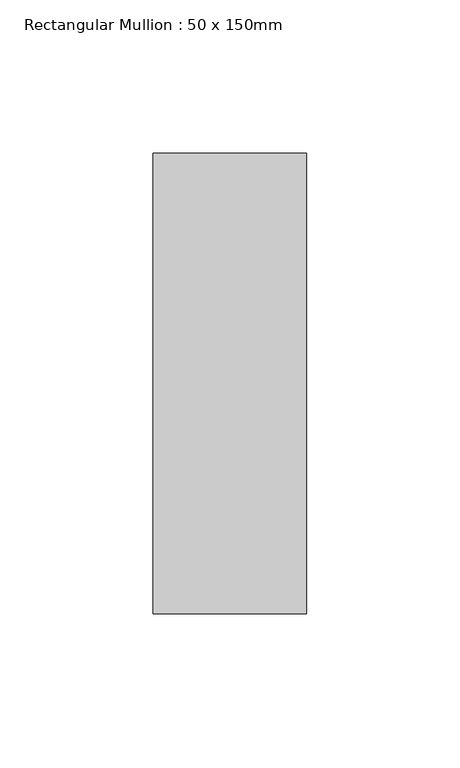
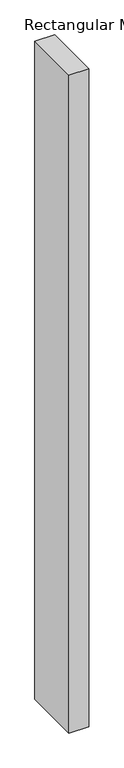
"""IFC4 building model written with IfcOpenShell, lengths in millimetres: member geometry, Rectangular Mullion : 50 x 150mm."""

import ifcopenshell
import ifcopenshell.guid

model = None  # the IFC model being written
_history = None  # IfcOwnerHistory: only IFC2X3 demands one
_inside = {}  # id of a spatial element -> (the spatial element, [elements in it])
_under = {}  # id of a project, library or spatial element -> (it, [spatial elements below it])
_declared = {}  # id of a project -> (the project, [libraries it declares])
_typed = {}  # id of a type object -> (the type object, [elements of that type])
_made_of = {}  # id of a material, layer set ... -> (it, [elements and type objects made of it])


def new_model(schema):
    """Start an empty IFC model of exactly this schema.

    Asked for "IFC4X3", IfcOpenShell would pick the latest addendum, in which some entities
    have other attributes; the version numbers below select the first issue.
    IFC2X3 requires an IfcOwnerHistory on every rooted entity: one is made here for all.
    """
    global model, _history
    if schema == "IFC4X3":
        model = ifcopenshell.file(schema_version=(4, 3, 0, 0))
    else:
        model = ifcopenshell.file(schema=schema)
    _inside.clear()
    _under.clear()
    _declared.clear()
    _typed.clear()
    _made_of.clear()
    _history = None
    if model.schema == "IFC2X3":
        org = make("IfcOrganization", Name="unknown")
        user = make(
            "IfcPersonAndOrganization",
            ThePerson=make("IfcPerson", FamilyName="unknown"),
            TheOrganization=org,
        )
        app = make(
            "IfcApplication",
            ApplicationDeveloper=org,
            Version="unknown",
            ApplicationFullName="unknown",
            ApplicationIdentifier="unknown",
        )
        _history = make(
            "IfcOwnerHistory",
            OwningUser=user,
            OwningApplication=app,
            ChangeAction="ADDED",
            CreationDate=0,
        )
    return model


def make(cls, **values):
    """One entity of the class cls with the attributes given. An attribute that is None is left unset."""
    return model.create_entity(
        cls, **{name: value for name, value in values.items() if value is not None}
    )


def rooted(cls, **values):
    """An entity with a GlobalId (a new one), such as an element, a storey or a relation."""
    return make(cls, GlobalId=ifcopenshell.guid.new(), OwnerHistory=_history, **values)


def si_unit(unit_type, name, prefix=None):
    """IfcSIUnit, for example si_unit("LENGTHUNIT", "METRE", prefix="MILLI")."""
    return make("IfcSIUnit", UnitType=unit_type, Prefix=prefix, Name=name)


def assignment(units):
    """IfcUnitAssignment: the units of a project."""
    return None if units is None else make("IfcUnitAssignment", Units=units)


def point(xyz):
    """IfcCartesianPoint."""
    return None if xyz is None else make("IfcCartesianPoint", Coordinates=xyz)


def direction(xyz):
    """IfcDirection."""
    return None if xyz is None else make("IfcDirection", DirectionRatios=xyz)


def frame(location, z_axis=None, x_axis=None):
    """IfcAxis2Placement3D, a coordinate frame: its origin and axes. An axis left out is left unset."""
    return make(
        "IfcAxis2Placement3D",
        Location=point(location),
        Axis=direction(z_axis),
        RefDirection=direction(x_axis),
    )


def origin():
    """The frame at (0, 0, 0) with its axes left unset."""
    return frame((0.0, 0.0, 0.0))


def place(relative_to, where):
    """IfcLocalPlacement: puts the frame where relative to a parent placement (None: the world)."""
    return make(
        "IfcLocalPlacement", PlacementRelTo=relative_to, RelativePlacement=where
    )


def context(
    kind, dimensions, precision=None, world=None, true_north=None, identifier=None
):
    """IfcGeometricRepresentationContext, for example the 3D "Model" context."""
    return make(
        "IfcGeometricRepresentationContext",
        ContextIdentifier=identifier,
        ContextType=kind,
        CoordinateSpaceDimension=dimensions,
        Precision=precision,
        WorldCoordinateSystem=world,
        TrueNorth=true_north,
    )


def project(units=None, contexts=None):
    """IfcProject with its units and contexts."""
    return rooted(
        "IfcProject",
        Name="project",
        RepresentationContexts=contexts,
        UnitsInContext=assignment(units),
    )


def spatial(cls, under=None, at=None, **own):
    """A site, building, storey or space (cls), placed at a placement, below another one or the project."""
    s = rooted(cls, ObjectPlacement=at, **own)
    if under is not None:
        _under.setdefault(under.id(), (under, []))[1].append(s)
    return s


def polyline(points):
    """IfcPolyline through the points."""
    return make("IfcPolyline", Points=[point(p) for p in points])


def outline(outer, holes=None, kind="AREA"):
    """IfcArbitraryClosedProfileDef: a profile drawn as a closed curve; with holes, ...WithVoids."""
    if holes is None:
        return make("IfcArbitraryClosedProfileDef", ProfileType=kind, OuterCurve=outer)
    return make(
        "IfcArbitraryProfileDefWithVoids",
        ProfileType=kind,
        OuterCurve=outer,
        InnerCurves=holes,
    )


def extrude(swept, where, along, depth):
    """IfcExtrudedAreaSolid: the profile swept, set in the frame where, extruded along a direction by depth."""
    return make(
        "IfcExtrudedAreaSolid",
        SweptArea=swept,
        Position=where,
        ExtrudedDirection=direction(along),
        Depth=depth,
    )


def shape(context_of_items, identifier, shape_type, items):
    """IfcShapeRepresentation: the items that make up one representation, for example the "Body"."""
    return make(
        "IfcShapeRepresentation",
        ContextOfItems=context_of_items,
        RepresentationIdentifier=identifier,
        RepresentationType=shape_type,
        Items=items,
    )


def source(mapping_origin, context_of_items, identifier, shape_type, items):
    """IfcRepresentationMap: a shape defined once, which mapped items show again and again."""
    return make(
        "IfcRepresentationMap",
        MappingOrigin=mapping_origin,
        MappedRepresentation=shape(context_of_items, identifier, shape_type, items),
    )


def transform(
    local_origin,
    x_axis=None,
    y_axis=None,
    z_axis=None,
    scale=None,
    scale2=None,
    scale3=None,
    uniform=True,
):
    """IfcCartesianTransformationOperator3D, or its non-uniform kind. x_axis, y_axis, z_axis: its Axis1, 2, 3."""
    if uniform:
        return make(
            "IfcCartesianTransformationOperator3D",
            Axis1=direction(x_axis),
            Axis2=direction(y_axis),
            LocalOrigin=point(local_origin),
            Scale=scale,
            Axis3=direction(z_axis),
        )
    return make(
        "IfcCartesianTransformationOperator3DnonUniform",
        Axis1=direction(x_axis),
        Axis2=direction(y_axis),
        LocalOrigin=point(local_origin),
        Scale=scale,
        Axis3=direction(z_axis),
        Scale2=scale2,
        Scale3=scale3,
    )


def mapped(mapping_source, mapping_target):
    """IfcMappedItem: shows the shape of a source again, moved by a transform."""
    return make(
        "IfcMappedItem", MappingSource=mapping_source, MappingTarget=mapping_target
    )


def made_of(thing, what):
    """Note that an element or type object is made of a material, layer set ...; save() writes the relation."""
    if what is not None:
        _made_of.setdefault(what.id(), (what, []))[1].append(thing)
    return thing


def element(
    cls,
    number,
    at=None,
    inside=None,
    cuts=None,
    type_object=None,
    material=None,
    context=None,
    identifier="Body",
    shape_type=None,
    held_by="IfcProductDefinitionShape",
    body=None,
    shapes=None,
    **own,
):
    """One element of the class cls, such as IfcWall. Its Tag is "e" and its number.

    at: its placement. inside: the storey or other place that contains it. cuts: it is an
    opening in that element (IfcRelVoidsElement). A single representation is given by context,
    identifier, shape_type and body (its items); several are given by shapes. held_by: the class
    of the entity that holds the representations. save() writes the other relations.
    """
    e = rooted(cls, Tag="e%d" % number, ObjectPlacement=at, **own)
    if body is not None:
        shapes = [shape(context, identifier, shape_type, body)]
    if shapes is not None:
        e.Representation = make(held_by, Representations=shapes)
    if inside is not None:
        _inside.setdefault(inside.id(), (inside, []))[1].append(e)
    if cuts is not None:
        rooted(
            "IfcRelVoidsElement", RelatingBuildingElement=cuts, RelatedOpeningElement=e
        )
    if type_object is not None:
        _typed.setdefault(type_object.id(), (type_object, []))[1].append(e)
    return made_of(e, material)


def aggregate(whole, parts):
    """IfcRelAggregates: a whole, such as a stair, and the parts it consists of."""
    return rooted("IfcRelAggregates", RelatingObject=whole, RelatedObjects=parts)


def save(model, path):
    """Write the relations noted so far, then the file.

    IfcRelAggregates (storeys below a building ...), IfcRelContainedInSpatialStructure (elements
    in a storey), IfcRelDefinesByType, IfcRelAssociatesMaterial and IfcRelDeclares: one each for
    every whole, place, type object, material and project.
    """
    for whole, parts in _under.values():
        aggregate(whole, parts)
    for where, things in _inside.values():
        rooted(
            "IfcRelContainedInSpatialStructure",
            RelatedElements=things,
            RelatingStructure=where,
        )
    for kind, things in _typed.values():
        rooted("IfcRelDefinesByType", RelatedObjects=things, RelatingType=kind)
    for what, things in _made_of.values():
        rooted("IfcRelAssociatesMaterial", RelatedObjects=things, RelatingMaterial=what)
    for by, libraries in _declared.values():
        rooted("IfcRelDeclares", RelatingContext=by, RelatedDefinitions=libraries)
    model.write(path)


def rectangular_mullion_50_x_150mm_41ec5d26(model_context):
    return source(origin(), model_context, "Body", "SweptSolid", [
        extrude(outline(polyline([(0.0, 75.0), (0.0, -75.0), (-50.0, -75.0), (-50.0, 75.0), (0.0, 75.0)])), frame((0.0, 0.0, -1767.0), z_axis=(0.0, 0.0, 1.0), x_axis=(1.0, 0.0, 0.0)), (0.0, 0.0, 1.0), 1767.0),
    ])


if __name__ == "__main__":
    model = new_model("IFC4")
    model_context = context("Model", 3, world=origin())
    ifc_project = project(units=[si_unit("LENGTHUNIT", "METRE", prefix="MILLI")], contexts=[model_context])
    site = spatial("IfcSite", under=ifc_project)
    building = spatial("IfcBuilding", under=site)
    placement = place(None, origin())
    rectangular_mullion_50_x_150mm_shape = rectangular_mullion_50_x_150mm_41ec5d26(model_context)
    element("IfcMember", 1, ObjectType="Rectangular Mullion : 50 x 150mm", at=placement, inside=building, context=model_context, shape_type="MappedRepresentation", body=[
        mapped(rectangular_mullion_50_x_150mm_shape, transform((0.0, 0.0, 0.0), x_axis=(1.0, 0.0, 0.0), y_axis=(0.0, 1.0, 0.0), z_axis=(0.0, 0.0, 1.0))),
    ])
    save(model, "model.ifc")

# Revit data of these elements
# Type "Rectangular Mullion : 50 x 150mm"
#   Keynote = "H11"
#   built-in parameter 1007304 = 0.492126 (stored number, unit not read)
#   built-in parameter 1007301 = 0.082021 (stored number, unit not read)
#   built-in parameter 1007300 = 0.082021 (stored number, unit not read)
# Element 1 (IfcMember, "Rectangular Mullion : 50 x 150mm")
#   Materials on its faces: "Aluminium"
# Materials
#   "Aluminium": class "Metal", colour RGB 247 247 247, transparency 0, Description = "Aluminium 6061", Cost = 0
